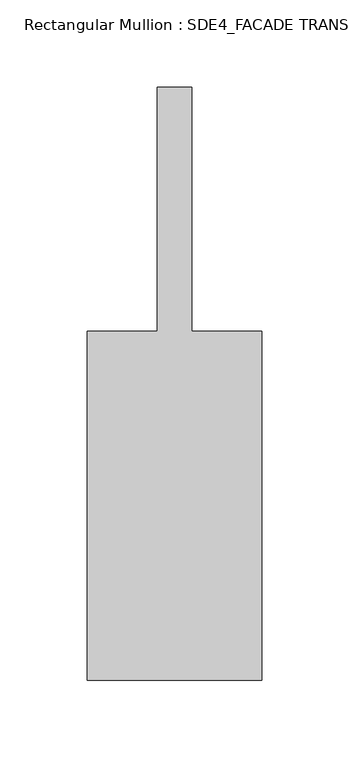
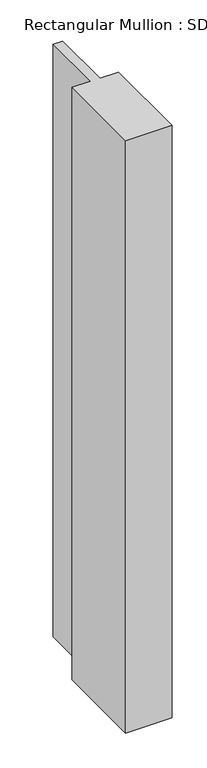
"""IFC4 building model written with IfcOpenShell, lengths in millimetres: member geometry, Rectangular Mullion : SDE4_FACADE TRANSOM TYPE 1."""

from ifc_helpers import new_model, si_unit, frame, origin, place, context, project, spatial, polyline, outline, extrude, source, transform, mapped, element, save


def rectangular_mullion_sde4_facade_transom_type_1_7de1c4af(model_context):
    return source(origin(), model_context, "Body", "SweptSolid", [
        extrude(outline(polyline([(50.0, -132.5), (-50.0, -132.5), (-50.0, 67.5), (-10.0, 67.5), (-10.0, 207.5), (10.0, 207.5), (10.0, 67.5), (50.0, 67.5), (50.0, -132.5)])), frame((0.0, 0.0, -1351.9884088), z_axis=(0.0, 0.0, 1.0), x_axis=(1.0, 0.0, 0.0)), (0.0, 0.0, 1.0), 1351.9884088),
    ])


if __name__ == "__main__":
    model = new_model("IFC4")
    model_context = context("Model", 3, world=origin())
    ifc_project = project(units=[si_unit("LENGTHUNIT", "METRE", prefix="MILLI")], contexts=[model_context])
    site = spatial("IfcSite", under=ifc_project)
    building = spatial("IfcBuilding", under=site)
    placement = place(None, origin())
    rectangular_mullion_sde4_facade_transom_type_1_shape = rectangular_mullion_sde4_facade_transom_type_1_7de1c4af(model_context)
    element("IfcMember", 1, ObjectType="Rectangular Mullion : SDE4_FACADE TRANSOM TYPE 1", at=placement, inside=building, context=model_context, shape_type="MappedRepresentation", body=[
        mapped(rectangular_mullion_sde4_facade_transom_type_1_shape, transform((0.0, 0.0, 0.0), x_axis=(1.0, 0.0, 0.0), y_axis=(0.0, 1.0, 0.0), z_axis=(0.0, 0.0, 1.0))),
    ])
    save(model, "model.ifc")

# Revit data of these elements
# Type "Rectangular Mullion : SDE4_FACADE TRANSOM TYPE 1"
#   built-in parameter 1007322 = 1.11549 (stored number, unit not read)
#   built-in parameter 1007321 = 0.164042 (stored number, unit not read)
#   built-in parameter 1007320 = 0.164042 (stored number, unit not read)
